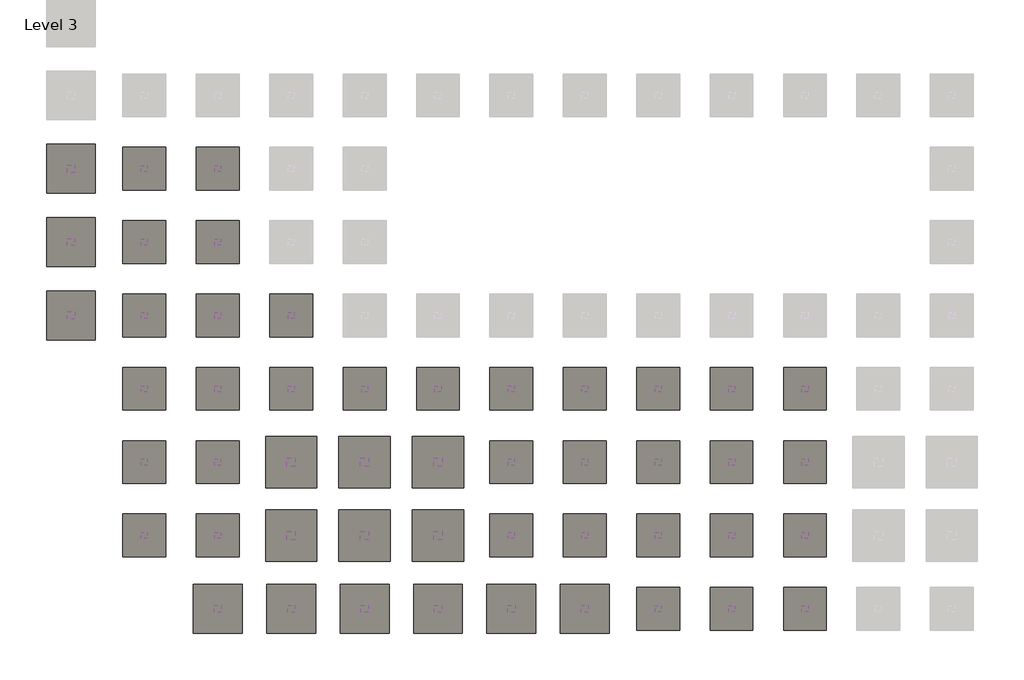
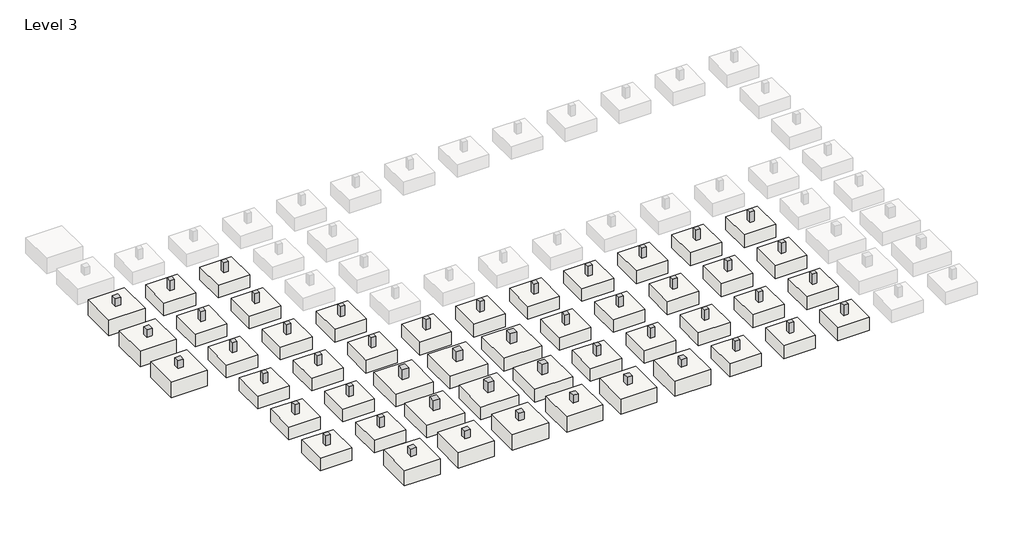
# One storey, part 1 of 3: 49 columns, 49 slabs.
"""IFC4 building model written with IfcOpenShell, lengths in millimetres."""

import ifcopenshell
import ifcopenshell.guid

model = None  # the IFC model being written
_history = None  # IfcOwnerHistory: only IFC2X3 demands one
_inside = {}  # id of a spatial element -> (the spatial element, [elements in it])
_under = {}  # id of a project, library or spatial element -> (it, [spatial elements below it])
_declared = {}  # id of a project -> (the project, [libraries it declares])
_typed = {}  # id of a type object -> (the type object, [elements of that type])
_made_of = {}  # id of a material, layer set ... -> (it, [elements and type objects made of it])


def new_model(schema):
    """Start an empty IFC model of exactly this schema.

    Asked for "IFC4X3", IfcOpenShell would pick the latest addendum, in which some entities
    have other attributes; the version numbers below select the first issue.
    IFC2X3 requires an IfcOwnerHistory on every rooted entity: one is made here for all.
    """
    global model, _history
    if schema == "IFC4X3":
        model = ifcopenshell.file(schema_version=(4, 3, 0, 0))
    else:
        model = ifcopenshell.file(schema=schema)
    _inside.clear()
    _under.clear()
    _declared.clear()
    _typed.clear()
    _made_of.clear()
    _history = None
    if model.schema == "IFC2X3":
        org = make("IfcOrganization", Name="unknown")
        user = make(
            "IfcPersonAndOrganization",
            ThePerson=make("IfcPerson", FamilyName="unknown"),
            TheOrganization=org,
        )
        app = make(
            "IfcApplication",
            ApplicationDeveloper=org,
            Version="unknown",
            ApplicationFullName="unknown",
            ApplicationIdentifier="unknown",
        )
        _history = make(
            "IfcOwnerHistory",
            OwningUser=user,
            OwningApplication=app,
            ChangeAction="ADDED",
            CreationDate=0,
        )
    return model


def make(cls, **values):
    """One entity of the class cls with the attributes given. An attribute that is None is left unset."""
    return model.create_entity(
        cls, **{name: value for name, value in values.items() if value is not None}
    )


def rooted(cls, **values):
    """An entity with a GlobalId (a new one), such as an element, a storey or a relation."""
    return make(cls, GlobalId=ifcopenshell.guid.new(), OwnerHistory=_history, **values)


def si_unit(unit_type, name, prefix=None):
    """IfcSIUnit, for example si_unit("LENGTHUNIT", "METRE", prefix="MILLI")."""
    return make("IfcSIUnit", UnitType=unit_type, Prefix=prefix, Name=name)


def assignment(units):
    """IfcUnitAssignment: the units of a project."""
    return None if units is None else make("IfcUnitAssignment", Units=units)


def point(xyz):
    """IfcCartesianPoint."""
    return None if xyz is None else make("IfcCartesianPoint", Coordinates=xyz)


def direction(xyz):
    """IfcDirection."""
    return None if xyz is None else make("IfcDirection", DirectionRatios=xyz)


def frame(location, z_axis=None, x_axis=None):
    """IfcAxis2Placement3D, a coordinate frame: its origin and axes. An axis left out is left unset."""
    return make(
        "IfcAxis2Placement3D",
        Location=point(location),
        Axis=direction(z_axis),
        RefDirection=direction(x_axis),
    )


def origin():
    """The frame at (0, 0, 0) with its axes left unset."""
    return frame((0.0, 0.0, 0.0))


def origin_with_axes():
    """The frame at (0, 0, 0) with the z axis (0, 0, 1) and the x axis (1, 0, 0) written out."""
    return frame((0.0, 0.0, 0.0), z_axis=(0.0, 0.0, 1.0), x_axis=(1.0, 0.0, 0.0))


def place(relative_to, where):
    """IfcLocalPlacement: puts the frame where relative to a parent placement (None: the world)."""
    return make(
        "IfcLocalPlacement", PlacementRelTo=relative_to, RelativePlacement=where
    )


def context(
    kind, dimensions, precision=None, world=None, true_north=None, identifier=None
):
    """IfcGeometricRepresentationContext, for example the 3D "Model" context."""
    return make(
        "IfcGeometricRepresentationContext",
        ContextIdentifier=identifier,
        ContextType=kind,
        CoordinateSpaceDimension=dimensions,
        Precision=precision,
        WorldCoordinateSystem=world,
        TrueNorth=true_north,
    )


def project(units=None, contexts=None):
    """IfcProject with its units and contexts."""
    return rooted(
        "IfcProject",
        Name="project",
        RepresentationContexts=contexts,
        UnitsInContext=assignment(units),
    )


def spatial(cls, under=None, at=None, **own):
    """A site, building, storey or space (cls), placed at a placement, below another one or the project."""
    s = rooted(cls, ObjectPlacement=at, **own)
    if under is not None:
        _under.setdefault(under.id(), (under, []))[1].append(s)
    return s


def polyline(points):
    """IfcPolyline through the points."""
    return make("IfcPolyline", Points=[point(p) for p in points])


def outline(outer, holes=None, kind="AREA"):
    """IfcArbitraryClosedProfileDef: a profile drawn as a closed curve; with holes, ...WithVoids."""
    if holes is None:
        return make("IfcArbitraryClosedProfileDef", ProfileType=kind, OuterCurve=outer)
    return make(
        "IfcArbitraryProfileDefWithVoids",
        ProfileType=kind,
        OuterCurve=outer,
        InnerCurves=holes,
    )


def extrude(swept, where, along, depth):
    """IfcExtrudedAreaSolid: the profile swept, set in the frame where, extruded along a direction by depth."""
    return make(
        "IfcExtrudedAreaSolid",
        SweptArea=swept,
        Position=where,
        ExtrudedDirection=direction(along),
        Depth=depth,
    )


def shape(context_of_items, identifier, shape_type, items):
    """IfcShapeRepresentation: the items that make up one representation, for example the "Body"."""
    return make(
        "IfcShapeRepresentation",
        ContextOfItems=context_of_items,
        RepresentationIdentifier=identifier,
        RepresentationType=shape_type,
        Items=items,
    )


def source(mapping_origin, context_of_items, identifier, shape_type, items):
    """IfcRepresentationMap: a shape defined once, which mapped items show again and again."""
    return make(
        "IfcRepresentationMap",
        MappingOrigin=mapping_origin,
        MappedRepresentation=shape(context_of_items, identifier, shape_type, items),
    )


def transform(
    local_origin,
    x_axis=None,
    y_axis=None,
    z_axis=None,
    scale=None,
    scale2=None,
    scale3=None,
    uniform=True,
):
    """IfcCartesianTransformationOperator3D, or its non-uniform kind. x_axis, y_axis, z_axis: its Axis1, 2, 3."""
    if uniform:
        return make(
            "IfcCartesianTransformationOperator3D",
            Axis1=direction(x_axis),
            Axis2=direction(y_axis),
            LocalOrigin=point(local_origin),
            Scale=scale,
            Axis3=direction(z_axis),
        )
    return make(
        "IfcCartesianTransformationOperator3DnonUniform",
        Axis1=direction(x_axis),
        Axis2=direction(y_axis),
        LocalOrigin=point(local_origin),
        Scale=scale,
        Axis3=direction(z_axis),
        Scale2=scale2,
        Scale3=scale3,
    )


def mapped(mapping_source, mapping_target):
    """IfcMappedItem: shows the shape of a source again, moved by a transform."""
    return make(
        "IfcMappedItem", MappingSource=mapping_source, MappingTarget=mapping_target
    )


def made_of(thing, what):
    """Note that an element or type object is made of a material, layer set ...; save() writes the relation."""
    if what is not None:
        _made_of.setdefault(what.id(), (what, []))[1].append(thing)
    return thing


def element(
    cls,
    number,
    at=None,
    inside=None,
    cuts=None,
    type_object=None,
    material=None,
    context=None,
    identifier="Body",
    shape_type=None,
    held_by="IfcProductDefinitionShape",
    body=None,
    shapes=None,
    **own,
):
    """One element of the class cls, such as IfcWall. Its Tag is "e" and its number.

    at: its placement. inside: the storey or other place that contains it. cuts: it is an
    opening in that element (IfcRelVoidsElement). A single representation is given by context,
    identifier, shape_type and body (its items); several are given by shapes. held_by: the class
    of the entity that holds the representations. save() writes the other relations.
    """
    e = rooted(cls, Tag="e%d" % number, ObjectPlacement=at, **own)
    if body is not None:
        shapes = [shape(context, identifier, shape_type, body)]
    if shapes is not None:
        e.Representation = make(held_by, Representations=shapes)
    if inside is not None:
        _inside.setdefault(inside.id(), (inside, []))[1].append(e)
    if cuts is not None:
        rooted(
            "IfcRelVoidsElement", RelatingBuildingElement=cuts, RelatedOpeningElement=e
        )
    if type_object is not None:
        _typed.setdefault(type_object.id(), (type_object, []))[1].append(e)
    return made_of(e, material)


def aggregate(whole, parts):
    """IfcRelAggregates: a whole, such as a stair, and the parts it consists of."""
    return rooted("IfcRelAggregates", RelatingObject=whole, RelatedObjects=parts)


def save(model, path):
    """Write the relations noted so far, then the file.

    IfcRelAggregates (storeys below a building ...), IfcRelContainedInSpatialStructure (elements
    in a storey), IfcRelDefinesByType, IfcRelAssociatesMaterial and IfcRelDeclares: one each for
    every whole, place, type object, material and project.
    """
    for whole, parts in _under.values():
        aggregate(whole, parts)
    for where, things in _inside.values():
        rooted(
            "IfcRelContainedInSpatialStructure",
            RelatedElements=things,
            RelatingStructure=where,
        )
    for kind, things in _typed.values():
        rooted("IfcRelDefinesByType", RelatedObjects=things, RelatingType=kind)
    for what, things in _made_of.values():
        rooted("IfcRelAssociatesMaterial", RelatedObjects=things, RelatingMaterial=what)
    for by, libraries in _declared.values():
        rooted("IfcRelDeclares", RelatingContext=by, RelatedDefinitions=libraries)
    model.write(path)


def cl111_concrete_rectangular_column_cl111_500x500_13a722a7(model_context):
    return source(origin(), model_context, "Body", "SweptSolid", [
        extrude(outline(polyline([(250.0, 250.0), (250.0, -250.0), (-250.0, -250.0), (-250.0, 250.0), (250.0, 250.0)])), frame((0.0, 0.0, -1200.0), z_axis=(0.0, 0.0, 1.0), x_axis=(1.0, 0.0, 0.0)), (0.0, 0.0, 1.0), 1200.0),
    ])


def cl111_concrete_rectangular_column_cl111_700x700_c1bab047(model_context):
    return source(origin(), model_context, "Body", "SweptSolid", [
        extrude(outline(polyline([(350.0, 350.0), (350.0, -350.0), (-350.0, -350.0), (-350.0, 350.0), (350.0, 350.0)])), frame((0.0, 0.0, -1200.0), z_axis=(0.0, 0.0, 1.0), x_axis=(1.0, 0.0, 0.0)), (0.0, 0.0, 1.0), 1200.0),
    ])


def ft111_footing_rectangular_ft111_3500x3500_d0491e67(model_context):
    return source(origin(), model_context, "Body", "SweptSolid", [
        extrude(outline(polyline([(1750.0, 1750.0), (1750.0, -1750.0), (-1750.0, -1750.0), (-1750.0, 1750.0), (1750.0, 1750.0)])), origin_with_axes(), (0.0, 0.0, 1.0), 1500.0),
    ])


def ft111_footing_rectangular_ft111_4200x4200_1dfe1a53(model_context):
    return source(origin(), model_context, "Body", "SweptSolid", [
        extrude(outline(polyline([(2100.0, 2100.0), (2100.0, -2100.0), (-2100.0, -2100.0), (-2100.0, 2100.0), (2100.0, 2100.0)])), origin_with_axes(), (0.0, 0.0, 1.0), 1500.0),
    ])


model = new_model("IFC4")

# Units and contexts
model_context = context("Model", 3, world=origin())
ifc_project = project(units=[si_unit("LENGTHUNIT", "METRE", prefix="MILLI")], contexts=[model_context])

# Site, building, storey
site = spatial("IfcSite", under=ifc_project)
building = spatial("IfcBuilding", under=site)
storey = spatial("IfcBuildingStorey", under=building, Name="Level 3", Elevation=-2700.0)

# Columns
placement = place(None, origin())
element("IfcColumn", 1, ObjectType="CL111_Concrete-Rectangular-Column : CL111_500x500", at=placement, inside=storey, context=model_context, shape_type="SweptSolid", body=[
    extrude(outline(polyline([(54250.0, -53750.0), (54250.0, -54250.0), (53750.0, -54250.0), (53750.0, -53750.0), (54250.0, -53750.0)])), frame((0.0, 0.0, -1200.0), z_axis=(0.0, 0.0, 1.0), x_axis=(1.0, 0.0, 0.0)), (0.0, 0.0, 1.0), 1200.0),
])
element("IfcColumn", 2, ObjectType="CL111_Concrete-Rectangular-Column : CL111_500x500", at=placement, inside=storey, context=model_context, shape_type="SweptSolid", body=[
    extrude(outline(polyline([(48250.0, -53750.0), (48250.0, -54250.0), (47750.0, -54250.0), (47750.0, -53750.0), (48250.0, -53750.0)])), frame((0.0, 0.0, -1200.0), z_axis=(0.0, 0.0, 1.0), x_axis=(1.0, 0.0, 0.0)), (0.0, 0.0, 1.0), 1200.0),
])
element("IfcColumn", 3, ObjectType="CL111_Concrete-Rectangular-Column : CL111_500x500", at=placement, inside=storey, context=model_context, shape_type="SweptSolid", body=[
    extrude(outline(polyline([(60250.0, -53750.0), (60250.0, -54250.0), (59750.0, -54250.0), (59750.0, -53750.0), (60250.0, -53750.0)])), frame((0.0, 0.0, -1200.0), z_axis=(0.0, 0.0, 1.0), x_axis=(1.0, 0.0, 0.0)), (0.0, 0.0, 1.0), 1200.0),
])
cl111_concrete_rectangular_column_cl111_500x500_shape = cl111_concrete_rectangular_column_cl111_500x500_13a722a7(model_context)
element("IfcColumn", 4, ObjectType="CL111_Concrete-Rectangular-Column : CL111_500x500", at=placement, inside=storey, context=model_context, shape_type="MappedRepresentation", body=[
    mapped(cl111_concrete_rectangular_column_cl111_500x500_shape, transform((54000.0, -36000.0, 0.0), x_axis=(1.0, 0.0, 0.0), y_axis=(0.0, 1.0, 0.0), z_axis=(0.0, 0.0, 1.0))),
])
element("IfcColumn", 5, ObjectType="CL111_Concrete-Rectangular-Column : CL111_500x500", at=placement, inside=storey, context=model_context, shape_type="MappedRepresentation", body=[
    mapped(cl111_concrete_rectangular_column_cl111_500x500_shape, transform((54000.0, -48000.0, 0.0), x_axis=(1.0, 0.0, 0.0), y_axis=(0.0, 1.0, 0.0), z_axis=(0.0, 0.0, 1.0))),
])
element("IfcColumn", 6, ObjectType="CL111_Concrete-Rectangular-Column : CL111_500x500", at=placement, inside=storey, context=model_context, shape_type="MappedRepresentation", body=[
    mapped(cl111_concrete_rectangular_column_cl111_500x500_shape, transform((54000.0, -42000.0, 0.0), x_axis=(1.0, 0.0, 0.0), y_axis=(0.0, 1.0, 0.0), z_axis=(0.0, 0.0, 1.0))),
])
element("IfcColumn", 7, ObjectType="CL111_Concrete-Rectangular-Column : CL111_500x500", at=placement, inside=storey, context=model_context, shape_type="MappedRepresentation", body=[
    mapped(cl111_concrete_rectangular_column_cl111_500x500_shape, transform((6000.0, -24000.0, 0.0), x_axis=(1.0, 0.0, 0.0), y_axis=(0.0, 1.0, 0.0), z_axis=(0.0, 0.0, 1.0))),
])
element("IfcColumn", 8, ObjectType="CL111_Concrete-Rectangular-Column : CL111_500x500", at=placement, inside=storey, context=model_context, shape_type="MappedRepresentation", body=[
    mapped(cl111_concrete_rectangular_column_cl111_500x500_shape, transform((12000.0, -24000.0, 0.0), x_axis=(1.0, 0.0, 0.0), y_axis=(0.0, 1.0, 0.0), z_axis=(0.0, 0.0, 1.0))),
])
element("IfcColumn", 9, ObjectType="CL111_Concrete-Rectangular-Column : CL111_500x500", at=placement, inside=storey, context=model_context, shape_type="MappedRepresentation", body=[
    mapped(cl111_concrete_rectangular_column_cl111_500x500_shape, transform((6000.0, -36000.0, 0.0), x_axis=(1.0, 0.0, 0.0), y_axis=(0.0, 1.0, 0.0), z_axis=(0.0, 0.0, 1.0))),
])
element("IfcColumn", 10, ObjectType="CL111_Concrete-Rectangular-Column : CL111_500x500", at=placement, inside=storey, context=model_context, shape_type="MappedRepresentation", body=[
    mapped(cl111_concrete_rectangular_column_cl111_500x500_shape, transform((12000.0, -36000.0, 0.0), x_axis=(1.0, 0.0, 0.0), y_axis=(0.0, 1.0, 0.0), z_axis=(0.0, 0.0, 1.0))),
])
element("IfcColumn", 11, ObjectType="CL111_Concrete-Rectangular-Column : CL111_500x500", at=placement, inside=storey, context=model_context, shape_type="MappedRepresentation", body=[
    mapped(cl111_concrete_rectangular_column_cl111_500x500_shape, transform((30000.0, -36000.0, 0.0), x_axis=(1.0, 0.0, 0.0), y_axis=(0.0, 1.0, 0.0), z_axis=(0.0, 0.0, 1.0))),
])
element("IfcColumn", 12, ObjectType="CL111_Concrete-Rectangular-Column : CL111_500x500", at=placement, inside=storey, context=model_context, shape_type="MappedRepresentation", body=[
    mapped(cl111_concrete_rectangular_column_cl111_500x500_shape, transform((36000.0, -36000.0, 0.0), x_axis=(1.0, 0.0, 0.0), y_axis=(0.0, 1.0, 0.0), z_axis=(0.0, 0.0, 1.0))),
])
element("IfcColumn", 13, ObjectType="CL111_Concrete-Rectangular-Column : CL111_500x500", at=placement, inside=storey, context=model_context, shape_type="MappedRepresentation", body=[
    mapped(cl111_concrete_rectangular_column_cl111_500x500_shape, transform((18000.0, -36000.0, 0.0), x_axis=(1.0, 0.0, 0.0), y_axis=(0.0, 1.0, 0.0), z_axis=(0.0, 0.0, 1.0))),
])
element("IfcColumn", 14, ObjectType="CL111_Concrete-Rectangular-Column : CL111_500x500", at=placement, inside=storey, context=model_context, shape_type="MappedRepresentation", body=[
    mapped(cl111_concrete_rectangular_column_cl111_500x500_shape, transform((24000.0, -36000.0, 0.0), x_axis=(1.0, 0.0, 0.0), y_axis=(0.0, 1.0, 0.0), z_axis=(0.0, 0.0, 1.0))),
])
element("IfcColumn", 15, ObjectType="CL111_Concrete-Rectangular-Column : CL111_500x500", at=placement, inside=storey, context=model_context, shape_type="MappedRepresentation", body=[
    mapped(cl111_concrete_rectangular_column_cl111_500x500_shape, transform((42000.0, -36000.0, 0.0), x_axis=(1.0, 0.0, 0.0), y_axis=(0.0, 1.0, 0.0), z_axis=(0.0, 0.0, 1.0))),
])
element("IfcColumn", 16, ObjectType="CL111_Concrete-Rectangular-Column : CL111_500x500", at=placement, inside=storey, context=model_context, shape_type="MappedRepresentation", body=[
    mapped(cl111_concrete_rectangular_column_cl111_500x500_shape, transform((48000.0, -36000.0, 0.0), x_axis=(1.0, 0.0, 0.0), y_axis=(0.0, 1.0, 0.0), z_axis=(0.0, 0.0, 1.0))),
])
element("IfcColumn", 17, ObjectType="CL111_Concrete-Rectangular-Column : CL111_500x500", at=placement, inside=storey, context=model_context, shape_type="MappedRepresentation", body=[
    mapped(cl111_concrete_rectangular_column_cl111_500x500_shape, transform((12000.0, -18000.0, 0.0), x_axis=(1.0, 0.0, 0.0), y_axis=(0.0, 1.0, 0.0), z_axis=(0.0, 0.0, 1.0))),
])
element("IfcColumn", 18, ObjectType="CL111_Concrete-Rectangular-Column : CL111_500x500", at=placement, inside=storey, context=model_context, shape_type="MappedRepresentation", body=[
    mapped(cl111_concrete_rectangular_column_cl111_500x500_shape, transform((6000.0, -18000.0, 0.0), x_axis=(1.0, 0.0, 0.0), y_axis=(0.0, 1.0, 0.0), z_axis=(0.0, 0.0, 1.0))),
])
element("IfcColumn", 19, ObjectType="CL111_Concrete-Rectangular-Column : CL111_500x500", at=placement, inside=storey, context=model_context, shape_type="MappedRepresentation", body=[
    mapped(cl111_concrete_rectangular_column_cl111_500x500_shape, transform((12000.0, -30000.0, 0.0), x_axis=(1.0, 0.0, 0.0), y_axis=(0.0, 1.0, 0.0), z_axis=(0.0, 0.0, 1.0))),
])
element("IfcColumn", 20, ObjectType="CL111_Concrete-Rectangular-Column : CL111_500x500", at=placement, inside=storey, context=model_context, shape_type="MappedRepresentation", body=[
    mapped(cl111_concrete_rectangular_column_cl111_500x500_shape, transform((6000.0, -30000.0, 0.0), x_axis=(1.0, 0.0, 0.0), y_axis=(0.0, 1.0, 0.0), z_axis=(0.0, 0.0, 1.0))),
])
element("IfcColumn", 21, ObjectType="CL111_Concrete-Rectangular-Column : CL111_500x500", at=placement, inside=storey, context=model_context, shape_type="MappedRepresentation", body=[
    mapped(cl111_concrete_rectangular_column_cl111_500x500_shape, transform((18000.0, -30000.0, 0.0), x_axis=(1.0, 0.0, 0.0), y_axis=(0.0, 1.0, 0.0), z_axis=(0.0, 0.0, 1.0))),
])
element("IfcColumn", 22, ObjectType="CL111_Concrete-Rectangular-Column : CL111_500x500", at=placement, inside=storey, context=model_context, shape_type="MappedRepresentation", body=[
    mapped(cl111_concrete_rectangular_column_cl111_500x500_shape, transform((42000.0, -48000.0, 0.0), x_axis=(1.0, 0.0, 0.0), y_axis=(0.0, 1.0, 0.0), z_axis=(0.0, 0.0, 1.0))),
])
element("IfcColumn", 23, ObjectType="CL111_Concrete-Rectangular-Column : CL111_500x500", at=placement, inside=storey, context=model_context, shape_type="MappedRepresentation", body=[
    mapped(cl111_concrete_rectangular_column_cl111_500x500_shape, transform((48000.0, -48000.0, 0.0), x_axis=(1.0, 0.0, 0.0), y_axis=(0.0, 1.0, 0.0), z_axis=(0.0, 0.0, 1.0))),
])
element("IfcColumn", 24, ObjectType="CL111_Concrete-Rectangular-Column : CL111_500x500", at=placement, inside=storey, context=model_context, shape_type="MappedRepresentation", body=[
    mapped(cl111_concrete_rectangular_column_cl111_500x500_shape, transform((36000.0, -48000.0, 0.0), x_axis=(1.0, 0.0, 0.0), y_axis=(0.0, 1.0, 0.0), z_axis=(0.0, 0.0, 1.0))),
])
element("IfcColumn", 25, ObjectType="CL111_Concrete-Rectangular-Column : CL111_500x500", at=placement, inside=storey, context=model_context, shape_type="MappedRepresentation", body=[
    mapped(cl111_concrete_rectangular_column_cl111_500x500_shape, transform((6000.0, -48000.0, 0.0), x_axis=(1.0, 0.0, 0.0), y_axis=(0.0, 1.0, 0.0), z_axis=(0.0, 0.0, 1.0))),
])
element("IfcColumn", 26, ObjectType="CL111_Concrete-Rectangular-Column : CL111_500x500", at=placement, inside=storey, context=model_context, shape_type="MappedRepresentation", body=[
    mapped(cl111_concrete_rectangular_column_cl111_500x500_shape, transform((12000.0, -48000.0, 0.0), x_axis=(1.0, 0.0, 0.0), y_axis=(0.0, 1.0, 0.0), z_axis=(0.0, 0.0, 1.0))),
])
element("IfcColumn", 27, ObjectType="CL111_Concrete-Rectangular-Column : CL111_500x500", at=placement, inside=storey, context=model_context, shape_type="MappedRepresentation", body=[
    mapped(cl111_concrete_rectangular_column_cl111_500x500_shape, transform((48000.0, -42000.0, 0.0), x_axis=(1.0, 0.0, 0.0), y_axis=(0.0, 1.0, 0.0), z_axis=(0.0, 0.0, 1.0))),
])
element("IfcColumn", 28, ObjectType="CL111_Concrete-Rectangular-Column : CL111_500x500", at=placement, inside=storey, context=model_context, shape_type="MappedRepresentation", body=[
    mapped(cl111_concrete_rectangular_column_cl111_500x500_shape, transform((42000.0, -42000.0, 0.0), x_axis=(1.0, 0.0, 0.0), y_axis=(0.0, 1.0, 0.0), z_axis=(0.0, 0.0, 1.0))),
])
element("IfcColumn", 29, ObjectType="CL111_Concrete-Rectangular-Column : CL111_500x500", at=placement, inside=storey, context=model_context, shape_type="MappedRepresentation", body=[
    mapped(cl111_concrete_rectangular_column_cl111_500x500_shape, transform((36000.0, -42000.0, 0.0), x_axis=(1.0, 0.0, 0.0), y_axis=(0.0, 1.0, 0.0), z_axis=(0.0, 0.0, 1.0))),
])
element("IfcColumn", 30, ObjectType="CL111_Concrete-Rectangular-Column : CL111_500x500", at=placement, inside=storey, context=model_context, shape_type="MappedRepresentation", body=[
    mapped(cl111_concrete_rectangular_column_cl111_500x500_shape, transform((12000.0, -42000.0, 0.0), x_axis=(1.0, 0.0, 0.0), y_axis=(0.0, 1.0, 0.0), z_axis=(0.0, 0.0, 1.0))),
])
element("IfcColumn", 31, ObjectType="CL111_Concrete-Rectangular-Column : CL111_500x500", at=placement, inside=storey, context=model_context, shape_type="MappedRepresentation", body=[
    mapped(cl111_concrete_rectangular_column_cl111_500x500_shape, transform((6000.0, -42000.0, 0.0), x_axis=(1.0, 0.0, 0.0), y_axis=(0.0, 1.0, 0.0), z_axis=(0.0, 0.0, 1.0))),
])
element("IfcColumn", 32, ObjectType="CL111_Concrete-Rectangular-Column : CL111_500x500", at=placement, inside=storey, context=model_context, shape_type="MappedRepresentation", body=[
    mapped(cl111_concrete_rectangular_column_cl111_500x500_shape, transform((60000.0, -36000.0, 0.0), x_axis=(1.0, 0.0, 0.0), y_axis=(0.0, 1.0, 0.0), z_axis=(0.0, 0.0, 1.0))),
])
element("IfcColumn", 33, ObjectType="CL111_Concrete-Rectangular-Column : CL111_500x500", at=placement, inside=storey, context=model_context, shape_type="MappedRepresentation", body=[
    mapped(cl111_concrete_rectangular_column_cl111_500x500_shape, transform((60000.0, -48000.0, 0.0), x_axis=(1.0, 0.0, 0.0), y_axis=(0.0, 1.0, 0.0), z_axis=(0.0, 0.0, 1.0))),
])
element("IfcColumn", 34, ObjectType="CL111_Concrete-Rectangular-Column : CL111_500x500", at=placement, inside=storey, context=model_context, shape_type="MappedRepresentation", body=[
    mapped(cl111_concrete_rectangular_column_cl111_500x500_shape, transform((60000.0, -42000.0, 0.0), x_axis=(1.0, 0.0, 0.0), y_axis=(0.0, 1.0, 0.0), z_axis=(0.0, 0.0, 1.0))),
])
element("IfcColumn", 35, ObjectType="CL111_Concrete-Rectangular-Column : CL111_600x600", at=placement, inside=storey, context=model_context, shape_type="SweptSolid", body=[
    extrude(outline(polyline([(300.0, -23700.0), (300.0, -24300.0), (-300.0, -24300.0), (-300.0, -23700.0), (300.0, -23700.0)])), frame((0.0, 0.0, -900.0), z_axis=(0.0, 0.0, 1.0), x_axis=(1.0, 0.0, 0.0)), (0.0, 0.0, 1.0), 900.0),
])
element("IfcColumn", 36, ObjectType="CL111_Concrete-Rectangular-Column : CL111_600x600", at=placement, inside=storey, context=model_context, shape_type="SweptSolid", body=[
    extrude(outline(polyline([(300.0, -17700.0), (300.0, -18300.0), (-300.0, -18300.0), (-300.0, -17700.0), (300.0, -17700.0)])), frame((0.0, 0.0, -900.0), z_axis=(0.0, 0.0, 1.0), x_axis=(1.0, 0.0, 0.0)), (0.0, 0.0, 1.0), 900.0),
])
element("IfcColumn", 37, ObjectType="CL111_Concrete-Rectangular-Column : CL111_600x600", at=placement, inside=storey, context=model_context, shape_type="SweptSolid", body=[
    extrude(outline(polyline([(300.0, -29700.0), (300.0, -30300.0), (-300.0, -30300.0), (-300.0, -29700.0), (300.0, -29700.0)])), frame((0.0, 0.0, -900.0), z_axis=(0.0, 0.0, 1.0), x_axis=(1.0, 0.0, 0.0)), (0.0, 0.0, 1.0), 900.0),
])
element("IfcColumn", 38, ObjectType="CL111_Concrete-Rectangular-Column : CL111_600x600", at=placement, inside=storey, context=model_context, shape_type="SweptSolid", body=[
    extrude(outline(polyline([(42300.0, -53700.0), (42300.0, -54300.0), (41700.0, -54300.0), (41700.0, -53700.0), (42300.0, -53700.0)])), frame((0.0, 0.0, -900.0), z_axis=(0.0, 0.0, 1.0), x_axis=(1.0, 0.0, 0.0)), (0.0, 0.0, 1.0), 900.0),
])
element("IfcColumn", 39, ObjectType="CL111_Concrete-Rectangular-Column : CL111_600x600", at=placement, inside=storey, context=model_context, shape_type="SweptSolid", body=[
    extrude(outline(polyline([(36300.0, -53700.0), (36300.0, -54300.0), (35700.0, -54300.0), (35700.0, -53700.0), (36300.0, -53700.0)])), frame((0.0, 0.0, -900.0), z_axis=(0.0, 0.0, 1.0), x_axis=(1.0, 0.0, 0.0)), (0.0, 0.0, 1.0), 900.0),
])
element("IfcColumn", 40, ObjectType="CL111_Concrete-Rectangular-Column : CL111_600x600", at=placement, inside=storey, context=model_context, shape_type="SweptSolid", body=[
    extrude(outline(polyline([(30300.0, -53700.0), (30300.0, -54300.0), (29700.0, -54300.0), (29700.0, -53700.0), (30300.0, -53700.0)])), frame((0.0, 0.0, -900.0), z_axis=(0.0, 0.0, 1.0), x_axis=(1.0, 0.0, 0.0)), (0.0, 0.0, 1.0), 900.0),
])
element("IfcColumn", 41, ObjectType="CL111_Concrete-Rectangular-Column : CL111_600x600", at=placement, inside=storey, context=model_context, shape_type="SweptSolid", body=[
    extrude(outline(polyline([(24300.0, -53700.0), (24300.0, -54300.0), (23700.0, -54300.0), (23700.0, -53700.0), (24300.0, -53700.0)])), frame((0.0, 0.0, -900.0), z_axis=(0.0, 0.0, 1.0), x_axis=(1.0, 0.0, 0.0)), (0.0, 0.0, 1.0), 900.0),
])
element("IfcColumn", 42, ObjectType="CL111_Concrete-Rectangular-Column : CL111_600x600", at=placement, inside=storey, context=model_context, shape_type="SweptSolid", body=[
    extrude(outline(polyline([(18300.0, -53700.0), (18300.0, -54300.0), (17700.0, -54300.0), (17700.0, -53700.0), (18300.0, -53700.0)])), frame((0.0, 0.0, -900.0), z_axis=(0.0, 0.0, 1.0), x_axis=(1.0, 0.0, 0.0)), (0.0, 0.0, 1.0), 900.0),
])
element("IfcColumn", 43, ObjectType="CL111_Concrete-Rectangular-Column : CL111_600x600", at=placement, inside=storey, context=model_context, shape_type="SweptSolid", body=[
    extrude(outline(polyline([(12300.0, -53700.0), (12300.0, -54300.0), (11700.0, -54300.0), (11700.0, -53700.0), (12300.0, -53700.0)])), frame((0.0, 0.0, -900.0), z_axis=(0.0, 0.0, 1.0), x_axis=(1.0, 0.0, 0.0)), (0.0, 0.0, 1.0), 900.0),
])
cl111_concrete_rectangular_column_cl111_700x700_shape = cl111_concrete_rectangular_column_cl111_700x700_c1bab047(model_context)
element("IfcColumn", 44, ObjectType="CL111_Concrete-Rectangular-Column : CL111_700x700", at=placement, inside=storey, context=model_context, shape_type="MappedRepresentation", body=[
    mapped(cl111_concrete_rectangular_column_cl111_700x700_shape, transform((18000.0, -48000.0, 0.0), x_axis=(1.0, 0.0, 0.0), y_axis=(0.0, 1.0, 0.0), z_axis=(0.0, 0.0, 1.0))),
])
element("IfcColumn", 45, ObjectType="CL111_Concrete-Rectangular-Column : CL111_700x700", at=placement, inside=storey, context=model_context, shape_type="MappedRepresentation", body=[
    mapped(cl111_concrete_rectangular_column_cl111_700x700_shape, transform((24000.0, -48000.0, 0.0), x_axis=(1.0, 0.0, 0.0), y_axis=(0.0, 1.0, 0.0), z_axis=(0.0, 0.0, 1.0))),
])
element("IfcColumn", 46, ObjectType="CL111_Concrete-Rectangular-Column : CL111_700x700", at=placement, inside=storey, context=model_context, shape_type="MappedRepresentation", body=[
    mapped(cl111_concrete_rectangular_column_cl111_700x700_shape, transform((30000.0, -48000.0, 0.0), x_axis=(1.0, 0.0, 0.0), y_axis=(0.0, 1.0, 0.0), z_axis=(0.0, 0.0, 1.0))),
])
element("IfcColumn", 47, ObjectType="CL111_Concrete-Rectangular-Column : CL111_700x700", at=placement, inside=storey, context=model_context, shape_type="MappedRepresentation", body=[
    mapped(cl111_concrete_rectangular_column_cl111_700x700_shape, transform((24000.0, -42000.0, 0.0), x_axis=(1.0, 0.0, 0.0), y_axis=(0.0, 1.0, 0.0), z_axis=(0.0, 0.0, 1.0))),
])
element("IfcColumn", 48, ObjectType="CL111_Concrete-Rectangular-Column : CL111_700x700", at=placement, inside=storey, context=model_context, shape_type="MappedRepresentation", body=[
    mapped(cl111_concrete_rectangular_column_cl111_700x700_shape, transform((18000.0, -42000.0, 0.0), x_axis=(1.0, 0.0, 0.0), y_axis=(0.0, 1.0, 0.0), z_axis=(0.0, 0.0, 1.0))),
])
element("IfcColumn", 49, ObjectType="CL111_Concrete-Rectangular-Column : CL111_700x700", at=placement, inside=storey, context=model_context, shape_type="MappedRepresentation", body=[
    mapped(cl111_concrete_rectangular_column_cl111_700x700_shape, transform((30000.0, -42000.0, 0.0), x_axis=(1.0, 0.0, 0.0), y_axis=(0.0, 1.0, 0.0), z_axis=(0.0, 0.0, 1.0))),
])

# Slabs
element("IfcSlab", 50, ObjectType="FT111_Footing-Rectangular : FT111_3500x3500", at=placement, inside=storey, context=model_context, shape_type="SweptSolid", body=[
    extrude(outline(polyline([(55750.0, -52250.0), (55750.0, -55750.0), (52250.0, -55750.0), (52250.0, -52250.0), (55750.0, -52250.0)])), frame((0.0, 0.0, -2700.0), z_axis=(0.0, 0.0, 1.0), x_axis=(1.0, 0.0, 0.0)), (0.0, 0.0, 1.0), 1500.0),
])
element("IfcSlab", 51, ObjectType="FT111_Footing-Rectangular : FT111_3500x3500", at=placement, inside=storey, context=model_context, shape_type="SweptSolid", body=[
    extrude(outline(polyline([(49750.0, -52250.0), (49750.0, -55750.0), (46250.0, -55750.0), (46250.0, -52250.0), (49750.0, -52250.0)])), frame((0.0, 0.0, -2700.0), z_axis=(0.0, 0.0, 1.0), x_axis=(1.0, 0.0, 0.0)), (0.0, 0.0, 1.0), 1500.0),
])
element("IfcSlab", 52, ObjectType="FT111_Footing-Rectangular : FT111_3500x3500", at=placement, inside=storey, context=model_context, shape_type="SweptSolid", body=[
    extrude(outline(polyline([(61750.0, -52250.0), (61750.0, -55750.0), (58250.0, -55750.0), (58250.0, -52250.0), (61750.0, -52250.0)])), frame((0.0, 0.0, -2700.0), z_axis=(0.0, 0.0, 1.0), x_axis=(1.0, 0.0, 0.0)), (0.0, 0.0, 1.0), 1500.0),
])
ft111_footing_rectangular_ft111_3500x3500_shape = ft111_footing_rectangular_ft111_3500x3500_d0491e67(model_context)
element("IfcSlab", 53, ObjectType="FT111_Footing-Rectangular : FT111_3500x3500", at=placement, inside=storey, context=model_context, shape_type="MappedRepresentation", body=[
    mapped(ft111_footing_rectangular_ft111_3500x3500_shape, transform((54000.0, -36000.0, -2700.0), x_axis=(1.0, 0.0, 0.0), y_axis=(0.0, 1.0, 0.0), z_axis=(0.0, 0.0, 1.0))),
])
element("IfcSlab", 54, ObjectType="FT111_Footing-Rectangular : FT111_3500x3500", at=placement, inside=storey, context=model_context, shape_type="MappedRepresentation", body=[
    mapped(ft111_footing_rectangular_ft111_3500x3500_shape, transform((54000.0, -48000.0, -2700.0), x_axis=(1.0, 0.0, 0.0), y_axis=(0.0, 1.0, 0.0), z_axis=(0.0, 0.0, 1.0))),
])
element("IfcSlab", 55, ObjectType="FT111_Footing-Rectangular : FT111_3500x3500", at=placement, inside=storey, context=model_context, shape_type="MappedRepresentation", body=[
    mapped(ft111_footing_rectangular_ft111_3500x3500_shape, transform((54000.0, -42000.0, -2700.0), x_axis=(1.0, 0.0, 0.0), y_axis=(0.0, 1.0, 0.0), z_axis=(0.0, 0.0, 1.0))),
])
element("IfcSlab", 56, ObjectType="FT111_Footing-Rectangular : FT111_3500x3500", at=placement, inside=storey, context=model_context, shape_type="MappedRepresentation", body=[
    mapped(ft111_footing_rectangular_ft111_3500x3500_shape, transform((6000.0, -24000.0, -2700.0), x_axis=(1.0, 0.0, 0.0), y_axis=(0.0, 1.0, 0.0), z_axis=(0.0, 0.0, 1.0))),
])
element("IfcSlab", 57, ObjectType="FT111_Footing-Rectangular : FT111_3500x3500", at=placement, inside=storey, context=model_context, shape_type="MappedRepresentation", body=[
    mapped(ft111_footing_rectangular_ft111_3500x3500_shape, transform((12000.0, -24000.0, -2700.0), x_axis=(1.0, 0.0, 0.0), y_axis=(0.0, 1.0, 0.0), z_axis=(0.0, 0.0, 1.0))),
])
element("IfcSlab", 58, ObjectType="FT111_Footing-Rectangular : FT111_3500x3500", at=placement, inside=storey, context=model_context, shape_type="MappedRepresentation", body=[
    mapped(ft111_footing_rectangular_ft111_3500x3500_shape, transform((6000.0, -36000.0, -2700.0), x_axis=(1.0, 0.0, 0.0), y_axis=(0.0, 1.0, 0.0), z_axis=(0.0, 0.0, 1.0))),
])
element("IfcSlab", 59, ObjectType="FT111_Footing-Rectangular : FT111_3500x3500", at=placement, inside=storey, context=model_context, shape_type="MappedRepresentation", body=[
    mapped(ft111_footing_rectangular_ft111_3500x3500_shape, transform((12000.0, -36000.0, -2700.0), x_axis=(1.0, 0.0, 0.0), y_axis=(0.0, 1.0, 0.0), z_axis=(0.0, 0.0, 1.0))),
])
element("IfcSlab", 60, ObjectType="FT111_Footing-Rectangular : FT111_3500x3500", at=placement, inside=storey, context=model_context, shape_type="MappedRepresentation", body=[
    mapped(ft111_footing_rectangular_ft111_3500x3500_shape, transform((30000.0, -36000.0, -2700.0), x_axis=(1.0, 0.0, 0.0), y_axis=(0.0, 1.0, 0.0), z_axis=(0.0, 0.0, 1.0))),
])
element("IfcSlab", 61, ObjectType="FT111_Footing-Rectangular : FT111_3500x3500", at=placement, inside=storey, context=model_context, shape_type="MappedRepresentation", body=[
    mapped(ft111_footing_rectangular_ft111_3500x3500_shape, transform((36000.0, -36000.0, -2700.0), x_axis=(1.0, 0.0, 0.0), y_axis=(0.0, 1.0, 0.0), z_axis=(0.0, 0.0, 1.0))),
])
element("IfcSlab", 62, ObjectType="FT111_Footing-Rectangular : FT111_3500x3500", at=placement, inside=storey, context=model_context, shape_type="MappedRepresentation", body=[
    mapped(ft111_footing_rectangular_ft111_3500x3500_shape, transform((18000.0, -36000.0, -2700.0), x_axis=(1.0, 0.0, 0.0), y_axis=(0.0, 1.0, 0.0), z_axis=(0.0, 0.0, 1.0))),
])
element("IfcSlab", 63, ObjectType="FT111_Footing-Rectangular : FT111_3500x3500", at=placement, inside=storey, context=model_context, shape_type="MappedRepresentation", body=[
    mapped(ft111_footing_rectangular_ft111_3500x3500_shape, transform((24000.0, -36000.0, -2700.0), x_axis=(1.0, 0.0, 0.0), y_axis=(0.0, 1.0, 0.0), z_axis=(0.0, 0.0, 1.0))),
])
element("IfcSlab", 64, ObjectType="FT111_Footing-Rectangular : FT111_3500x3500", at=placement, inside=storey, context=model_context, shape_type="MappedRepresentation", body=[
    mapped(ft111_footing_rectangular_ft111_3500x3500_shape, transform((42000.0, -36000.0, -2700.0), x_axis=(1.0, 0.0, 0.0), y_axis=(0.0, 1.0, 0.0), z_axis=(0.0, 0.0, 1.0))),
])
element("IfcSlab", 65, ObjectType="FT111_Footing-Rectangular : FT111_3500x3500", at=placement, inside=storey, context=model_context, shape_type="MappedRepresentation", body=[
    mapped(ft111_footing_rectangular_ft111_3500x3500_shape, transform((48000.0, -36000.0, -2700.0), x_axis=(1.0, 0.0, 0.0), y_axis=(0.0, 1.0, 0.0), z_axis=(0.0, 0.0, 1.0))),
])
element("IfcSlab", 66, ObjectType="FT111_Footing-Rectangular : FT111_3500x3500", at=placement, inside=storey, context=model_context, shape_type="MappedRepresentation", body=[
    mapped(ft111_footing_rectangular_ft111_3500x3500_shape, transform((12000.0, -18000.0, -2700.0), x_axis=(1.0, 0.0, 0.0), y_axis=(0.0, 1.0, 0.0), z_axis=(0.0, 0.0, 1.0))),
])
element("IfcSlab", 67, ObjectType="FT111_Footing-Rectangular : FT111_3500x3500", at=placement, inside=storey, context=model_context, shape_type="MappedRepresentation", body=[
    mapped(ft111_footing_rectangular_ft111_3500x3500_shape, transform((6000.0, -18000.0, -2700.0), x_axis=(1.0, 0.0, 0.0), y_axis=(0.0, 1.0, 0.0), z_axis=(0.0, 0.0, 1.0))),
])
element("IfcSlab", 68, ObjectType="FT111_Footing-Rectangular : FT111_3500x3500", at=placement, inside=storey, context=model_context, shape_type="MappedRepresentation", body=[
    mapped(ft111_footing_rectangular_ft111_3500x3500_shape, transform((12000.0, -30000.0, -2700.0), x_axis=(1.0, 0.0, 0.0), y_axis=(0.0, 1.0, 0.0), z_axis=(0.0, 0.0, 1.0))),
])
element("IfcSlab", 69, ObjectType="FT111_Footing-Rectangular : FT111_3500x3500", at=placement, inside=storey, context=model_context, shape_type="MappedRepresentation", body=[
    mapped(ft111_footing_rectangular_ft111_3500x3500_shape, transform((6000.0, -30000.0, -2700.0), x_axis=(1.0, 0.0, 0.0), y_axis=(0.0, 1.0, 0.0), z_axis=(0.0, 0.0, 1.0))),
])
element("IfcSlab", 70, ObjectType="FT111_Footing-Rectangular : FT111_3500x3500", at=placement, inside=storey, context=model_context, shape_type="MappedRepresentation", body=[
    mapped(ft111_footing_rectangular_ft111_3500x3500_shape, transform((18000.0, -30000.0, -2700.0), x_axis=(1.0, 0.0, 0.0), y_axis=(0.0, 1.0, 0.0), z_axis=(0.0, 0.0, 1.0))),
])
element("IfcSlab", 71, ObjectType="FT111_Footing-Rectangular : FT111_3500x3500", at=placement, inside=storey, context=model_context, shape_type="MappedRepresentation", body=[
    mapped(ft111_footing_rectangular_ft111_3500x3500_shape, transform((42000.0, -48000.0, -2700.0), x_axis=(1.0, 0.0, 0.0), y_axis=(0.0, 1.0, 0.0), z_axis=(0.0, 0.0, 1.0))),
])
element("IfcSlab", 72, ObjectType="FT111_Footing-Rectangular : FT111_3500x3500", at=placement, inside=storey, context=model_context, shape_type="MappedRepresentation", body=[
    mapped(ft111_footing_rectangular_ft111_3500x3500_shape, transform((48000.0, -48000.0, -2700.0), x_axis=(1.0, 0.0, 0.0), y_axis=(0.0, 1.0, 0.0), z_axis=(0.0, 0.0, 1.0))),
])
element("IfcSlab", 73, ObjectType="FT111_Footing-Rectangular : FT111_3500x3500", at=placement, inside=storey, context=model_context, shape_type="MappedRepresentation", body=[
    mapped(ft111_footing_rectangular_ft111_3500x3500_shape, transform((36000.0, -48000.0, -2700.0), x_axis=(1.0, 0.0, 0.0), y_axis=(0.0, 1.0, 0.0), z_axis=(0.0, 0.0, 1.0))),
])
element("IfcSlab", 74, ObjectType="FT111_Footing-Rectangular : FT111_3500x3500", at=placement, inside=storey, context=model_context, shape_type="MappedRepresentation", body=[
    mapped(ft111_footing_rectangular_ft111_3500x3500_shape, transform((6000.0, -48000.0, -2700.0), x_axis=(1.0, 0.0, 0.0), y_axis=(0.0, 1.0, 0.0), z_axis=(0.0, 0.0, 1.0))),
])
element("IfcSlab", 75, ObjectType="FT111_Footing-Rectangular : FT111_3500x3500", at=placement, inside=storey, context=model_context, shape_type="MappedRepresentation", body=[
    mapped(ft111_footing_rectangular_ft111_3500x3500_shape, transform((12000.0, -48000.0, -2700.0), x_axis=(1.0, 0.0, 0.0), y_axis=(0.0, 1.0, 0.0), z_axis=(0.0, 0.0, 1.0))),
])
element("IfcSlab", 76, ObjectType="FT111_Footing-Rectangular : FT111_3500x3500", at=placement, inside=storey, context=model_context, shape_type="MappedRepresentation", body=[
    mapped(ft111_footing_rectangular_ft111_3500x3500_shape, transform((48000.0, -42000.0, -2700.0), x_axis=(1.0, 0.0, 0.0), y_axis=(0.0, 1.0, 0.0), z_axis=(0.0, 0.0, 1.0))),
])
element("IfcSlab", 77, ObjectType="FT111_Footing-Rectangular : FT111_3500x3500", at=placement, inside=storey, context=model_context, shape_type="MappedRepresentation", body=[
    mapped(ft111_footing_rectangular_ft111_3500x3500_shape, transform((42000.0, -42000.0, -2700.0), x_axis=(1.0, 0.0, 0.0), y_axis=(0.0, 1.0, 0.0), z_axis=(0.0, 0.0, 1.0))),
])
element("IfcSlab", 78, ObjectType="FT111_Footing-Rectangular : FT111_3500x3500", at=placement, inside=storey, context=model_context, shape_type="MappedRepresentation", body=[
    mapped(ft111_footing_rectangular_ft111_3500x3500_shape, transform((36000.0, -42000.0, -2700.0), x_axis=(1.0, 0.0, 0.0), y_axis=(0.0, 1.0, 0.0), z_axis=(0.0, 0.0, 1.0))),
])
element("IfcSlab", 79, ObjectType="FT111_Footing-Rectangular : FT111_3500x3500", at=placement, inside=storey, context=model_context, shape_type="MappedRepresentation", body=[
    mapped(ft111_footing_rectangular_ft111_3500x3500_shape, transform((12000.0, -42000.0, -2700.0), x_axis=(1.0, 0.0, 0.0), y_axis=(0.0, 1.0, 0.0), z_axis=(0.0, 0.0, 1.0))),
])
element("IfcSlab", 80, ObjectType="FT111_Footing-Rectangular : FT111_3500x3500", at=placement, inside=storey, context=model_context, shape_type="MappedRepresentation", body=[
    mapped(ft111_footing_rectangular_ft111_3500x3500_shape, transform((6000.0, -42000.0, -2700.0), x_axis=(1.0, 0.0, 0.0), y_axis=(0.0, 1.0, 0.0), z_axis=(0.0, 0.0, 1.0))),
])
element("IfcSlab", 81, ObjectType="FT111_Footing-Rectangular : FT111_3500x3500", at=placement, inside=storey, context=model_context, shape_type="MappedRepresentation", body=[
    mapped(ft111_footing_rectangular_ft111_3500x3500_shape, transform((60000.0, -36000.0, -2700.0), x_axis=(1.0, 0.0, 0.0), y_axis=(0.0, 1.0, 0.0), z_axis=(0.0, 0.0, 1.0))),
])
element("IfcSlab", 82, ObjectType="FT111_Footing-Rectangular : FT111_3500x3500", at=placement, inside=storey, context=model_context, shape_type="MappedRepresentation", body=[
    mapped(ft111_footing_rectangular_ft111_3500x3500_shape, transform((60000.0, -48000.0, -2700.0), x_axis=(1.0, 0.0, 0.0), y_axis=(0.0, 1.0, 0.0), z_axis=(0.0, 0.0, 1.0))),
])
element("IfcSlab", 83, ObjectType="FT111_Footing-Rectangular : FT111_3500x3500", at=placement, inside=storey, context=model_context, shape_type="MappedRepresentation", body=[
    mapped(ft111_footing_rectangular_ft111_3500x3500_shape, transform((60000.0, -42000.0, -2700.0), x_axis=(1.0, 0.0, 0.0), y_axis=(0.0, 1.0, 0.0), z_axis=(0.0, 0.0, 1.0))),
])
element("IfcSlab", 84, ObjectType="FT111_Footing-Rectangular : FT111_4000x4000", at=placement, inside=storey, context=model_context, shape_type="SweptSolid", body=[
    extrude(outline(polyline([(2000.0, -22000.0), (2000.0, -26000.0), (-2000.0, -26000.0), (-2000.0, -22000.0), (2000.0, -22000.0)])), frame((0.0, 0.0, -2700.0), z_axis=(0.0, 0.0, 1.0), x_axis=(1.0, 0.0, 0.0)), (0.0, 0.0, 1.0), 1800.0),
])
element("IfcSlab", 85, ObjectType="FT111_Footing-Rectangular : FT111_4000x4000", at=placement, inside=storey, context=model_context, shape_type="SweptSolid", body=[
    extrude(outline(polyline([(2000.0, -16000.0), (2000.0, -20000.0), (-2000.0, -20000.0), (-2000.0, -16000.0), (2000.0, -16000.0)])), frame((0.0, 0.0, -2700.0), z_axis=(0.0, 0.0, 1.0), x_axis=(1.0, 0.0, 0.0)), (0.0, 0.0, 1.0), 1800.0),
])
element("IfcSlab", 86, ObjectType="FT111_Footing-Rectangular : FT111_4000x4000", at=placement, inside=storey, context=model_context, shape_type="SweptSolid", body=[
    extrude(outline(polyline([(2000.0, -28000.0), (2000.0, -32000.0), (-2000.0, -32000.0), (-2000.0, -28000.0), (2000.0, -28000.0)])), frame((0.0, 0.0, -2700.0), z_axis=(0.0, 0.0, 1.0), x_axis=(1.0, 0.0, 0.0)), (0.0, 0.0, 1.0), 1800.0),
])
element("IfcSlab", 87, ObjectType="FT111_Footing-Rectangular : FT111_4000x4000", at=placement, inside=storey, context=model_context, shape_type="SweptSolid", body=[
    extrude(outline(polyline([(44000.0, -52000.0), (44000.0, -56000.0), (40000.0, -56000.0), (40000.0, -52000.0), (44000.0, -52000.0)])), frame((0.0, 0.0, -2700.0), z_axis=(0.0, 0.0, 1.0), x_axis=(1.0, 0.0, 0.0)), (0.0, 0.0, 1.0), 1800.0),
])
element("IfcSlab", 88, ObjectType="FT111_Footing-Rectangular : FT111_4000x4000", at=placement, inside=storey, context=model_context, shape_type="SweptSolid", body=[
    extrude(outline(polyline([(38000.0, -52000.0), (38000.0, -56000.0), (34000.0, -56000.0), (34000.0, -52000.0), (38000.0, -52000.0)])), frame((0.0, 0.0, -2700.0), z_axis=(0.0, 0.0, 1.0), x_axis=(1.0, 0.0, 0.0)), (0.0, 0.0, 1.0), 1800.0),
])
element("IfcSlab", 89, ObjectType="FT111_Footing-Rectangular : FT111_4000x4000", at=placement, inside=storey, context=model_context, shape_type="SweptSolid", body=[
    extrude(outline(polyline([(32000.0, -52000.0), (32000.0, -56000.0), (28000.0, -56000.0), (28000.0, -52000.0), (32000.0, -52000.0)])), frame((0.0, 0.0, -2700.0), z_axis=(0.0, 0.0, 1.0), x_axis=(1.0, 0.0, 0.0)), (0.0, 0.0, 1.0), 1800.0),
])
element("IfcSlab", 90, ObjectType="FT111_Footing-Rectangular : FT111_4000x4000", at=placement, inside=storey, context=model_context, shape_type="SweptSolid", body=[
    extrude(outline(polyline([(26000.0, -52000.0), (26000.0, -56000.0), (22000.0, -56000.0), (22000.0, -52000.0), (26000.0, -52000.0)])), frame((0.0, 0.0, -2700.0), z_axis=(0.0, 0.0, 1.0), x_axis=(1.0, 0.0, 0.0)), (0.0, 0.0, 1.0), 1800.0),
])
element("IfcSlab", 91, ObjectType="FT111_Footing-Rectangular : FT111_4000x4000", at=placement, inside=storey, context=model_context, shape_type="SweptSolid", body=[
    extrude(outline(polyline([(20000.0, -52000.0), (20000.0, -56000.0), (16000.0, -56000.0), (16000.0, -52000.0), (20000.0, -52000.0)])), frame((0.0, 0.0, -2700.0), z_axis=(0.0, 0.0, 1.0), x_axis=(1.0, 0.0, 0.0)), (0.0, 0.0, 1.0), 1800.0),
])
element("IfcSlab", 92, ObjectType="FT111_Footing-Rectangular : FT111_4000x4000", at=placement, inside=storey, context=model_context, shape_type="SweptSolid", body=[
    extrude(outline(polyline([(14000.0, -52000.0), (14000.0, -56000.0), (10000.0, -56000.0), (10000.0, -52000.0), (14000.0, -52000.0)])), frame((0.0, 0.0, -2700.0), z_axis=(0.0, 0.0, 1.0), x_axis=(1.0, 0.0, 0.0)), (0.0, 0.0, 1.0), 1800.0),
])
ft111_footing_rectangular_ft111_4200x4200_shape = ft111_footing_rectangular_ft111_4200x4200_1dfe1a53(model_context)
element("IfcSlab", 93, ObjectType="FT111_Footing-Rectangular : FT111_4200x4200", at=placement, inside=storey, context=model_context, shape_type="MappedRepresentation", body=[
    mapped(ft111_footing_rectangular_ft111_4200x4200_shape, transform((18000.0, -48000.0, -2700.0), x_axis=(1.0, 0.0, 0.0), y_axis=(0.0, 1.0, 0.0), z_axis=(0.0, 0.0, 1.0))),
])
element("IfcSlab", 94, ObjectType="FT111_Footing-Rectangular : FT111_4200x4200", at=placement, inside=storey, context=model_context, shape_type="MappedRepresentation", body=[
    mapped(ft111_footing_rectangular_ft111_4200x4200_shape, transform((24000.0, -48000.0, -2700.0), x_axis=(1.0, 0.0, 0.0), y_axis=(0.0, 1.0, 0.0), z_axis=(0.0, 0.0, 1.0))),
])
element("IfcSlab", 95, ObjectType="FT111_Footing-Rectangular : FT111_4200x4200", at=placement, inside=storey, context=model_context, shape_type="MappedRepresentation", body=[
    mapped(ft111_footing_rectangular_ft111_4200x4200_shape, transform((30000.0, -48000.0, -2700.0), x_axis=(1.0, 0.0, 0.0), y_axis=(0.0, 1.0, 0.0), z_axis=(0.0, 0.0, 1.0))),
])
element("IfcSlab", 96, ObjectType="FT111_Footing-Rectangular : FT111_4200x4200", at=placement, inside=storey, context=model_context, shape_type="MappedRepresentation", body=[
    mapped(ft111_footing_rectangular_ft111_4200x4200_shape, transform((24000.0, -42000.0, -2700.0), x_axis=(1.0, 0.0, 0.0), y_axis=(0.0, 1.0, 0.0), z_axis=(0.0, 0.0, 1.0))),
])
element("IfcSlab", 97, ObjectType="FT111_Footing-Rectangular : FT111_4200x4200", at=placement, inside=storey, context=model_context, shape_type="MappedRepresentation", body=[
    mapped(ft111_footing_rectangular_ft111_4200x4200_shape, transform((18000.0, -42000.0, -2700.0), x_axis=(1.0, 0.0, 0.0), y_axis=(0.0, 1.0, 0.0), z_axis=(0.0, 0.0, 1.0))),
])
element("IfcSlab", 98, ObjectType="FT111_Footing-Rectangular : FT111_4200x4200", at=placement, inside=storey, context=model_context, shape_type="MappedRepresentation", body=[
    mapped(ft111_footing_rectangular_ft111_4200x4200_shape, transform((30000.0, -42000.0, -2700.0), x_axis=(1.0, 0.0, 0.0), y_axis=(0.0, 1.0, 0.0), z_axis=(0.0, 0.0, 1.0))),
])

save(model, "model.ifc")

# Revit data of these elements
# Project information
#   Project Issue Date = "Issue Date"
#   Project Status = "Project Status"
#   Client Name = "Owner"
#   Project Address = "Enter address here"
#   Project Name = "Project Name"
#   Project Number = "0001"
# Grids (mm)
#   "A": line (-6000, 0) -> (102000, 0)
#   "B": line (-6000, -6000) -> (102000, -6000)
#   "C": line (-6000, -12000) -> (102000, -12000)
#   "D": line (-6000, -18000) -> (102000, -18000)
#   "E": line (-6000, -24000) -> (102000, -24000)
#   "F": line (-6000, -30000) -> (102000, -30000)
#   "G": line (-6000, -36000) -> (102000, -36000)
#   "H": line (-6000, -42000) -> (102000, -42000)
#   "I": line (-6000, -48000) -> (102000, -48000)
#   "J": line (-6000, -54000) -> (102000, -54000)
#   "1": line (0, 6000) -> (0, -60000)
#   "2": line (6000, 6000) -> (6000, -60000)
#   "3": line (12000, 6000) -> (12000, -60000)
#   "4": line (18000, 6000) -> (18000, -60000)
#   "5": line (24000, 6000) -> (24000, -60000)
#   "6": line (30000, 6000) -> (30000, -60000)
#   "7": line (36000, 6000) -> (36000, -60000)
#   "8": line (42000, 6000) -> (42000, -60000)
#   "9": line (48000, 6000) -> (48000, -60000)
#   "10": line (54000, 6000) -> (54000, -60000)
#   "11": line (60000, 6000) -> (60000, -60000)
#   "12": line (66000, 6000) -> (66000, -60000)
#   "13": line (72000, 6000) -> (72000, -60000)
#   "14": line (78000, 6000) -> (78000, -60000)
#   "15": line (84000, 6000) -> (84000, -60000)
#   "16": line (90000, 6000) -> (90000, -60000)
#   "17": line (96000, 6000) -> (96000, -60000)
# Type "CL111_Concrete-Rectangular-Column : CL111_500x500"
#   Assembly Code = "B10"
#   b = 500 mm
#   h = 500 mm
#   Structural Material [instance default] = Concrete, Cast-in-Place gray
# Type "CL111_Concrete-Rectangular-Column : CL111_600x600"
#   Assembly Code = "B10"
#   b = 600 mm
#   h = 600 mm
#   Structural Material [instance default] = Concrete, Cast-in-Place gray
# Type "CL111_Concrete-Rectangular-Column : CL111_700x700"
#   Assembly Code = "B10"
#   b = 700 mm
#   h = 700 mm
#   Structural Material [instance default] = Concrete, Cast-in-Place gray
# Type "FT111_Footing-Rectangular : FT111_3500x3500"
#   Assembly Code = "A1010100"
#   Width = 3500 mm
#   Length = 3500 mm
#   Foundation Thickness = 1500 mm
#   Structural Material [instance default] = Concrete, Cast-in-Place gray
# Type "FT111_Footing-Rectangular : FT111_4000x4000"
#   Assembly Code = "A1010100"
#   Width = 4000 mm
#   Length = 4000 mm
#   Foundation Thickness = 1800 mm
#   Structural Material [instance default] = Concrete, Cast-in-Place gray
# Type "FT111_Footing-Rectangular : FT111_4200x4200"
#   Assembly Code = "A1010100"
#   Width = 4200 mm
#   Length = 4200 mm
#   Foundation Thickness = 1500 mm
#   Structural Material [instance default] = Concrete, Cast-in-Place gray
# Elements 1, 2, 3, 4, 5, 6, 7, 8, 9, 10, 11, 12, 13, 14, 15, 16, 17, 18, 19, 20, 21, 22, 23, 24, 25, 26, 27, 28, 29, 30, 31, 32, 33, 34 (IfcColumn, "CL111_Concrete-Rectangular-Column : CL111_500x500")
#   Structural Material = Concrete, Cast-in-Place gray
#   Phase Created = New Construction
#   Materials on its faces: "Concrete, Cast-in-Place gray"
# Elements 35, 36, 37, 38, 39, 40, 41, 42, 43 (IfcColumn, "CL111_Concrete-Rectangular-Column : CL111_600x600")
#   Structural Material = Concrete, Cast-in-Place gray
#   Phase Created = New Construction
#   Materials on its faces: "Concrete, Cast-in-Place gray"
# Elements 44, 45, 46, 47, 48, 49 (IfcColumn, "CL111_Concrete-Rectangular-Column : CL111_700x700")
#   Structural Material = Concrete, Cast-in-Place gray
#   Phase Created = New Construction
#   Materials on its faces: "Concrete, Cast-in-Place gray"
# Elements 50, 51, 52, 53, 54, 55, 56, 57, 58, 59, 60, 61, 62, 63, 64, 65, 66, 67, 68, 69, 70, 71, 72, 73, 74, 75, 76, 77, 78, 79, 80, 81, 82, 83 (IfcSlab, "FT111_Footing-Rectangular : FT111_3500x3500")
#   Structural Material = Concrete, Cast-in-Place gray
#   Phase Created = New Construction
#   Materials on its faces: "Concrete, Cast-in-Place gray"
# Elements 84, 85, 86, 87, 88, 89, 90, 91, 92 (IfcSlab, "FT111_Footing-Rectangular : FT111_4000x4000")
#   Structural Material = Concrete, Cast-in-Place gray
#   Phase Created = New Construction
#   Materials on its faces: "Concrete, Cast-in-Place gray"
# Elements 93, 94, 95, 96, 97, 98 (IfcSlab, "FT111_Footing-Rectangular : FT111_4200x4200")
#   Structural Material = Concrete, Cast-in-Place gray
#   Phase Created = New Construction
#   Materials on its faces: "Concrete, Cast-in-Place gray"
# Materials
#   "Concrete, Cast-in-Place gray": class "Concrete", colour RGB 192 192 192, transparency 0, Description = "Cast-in-place concrete", Cost = 0
